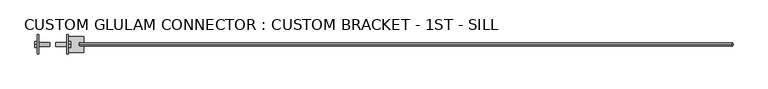
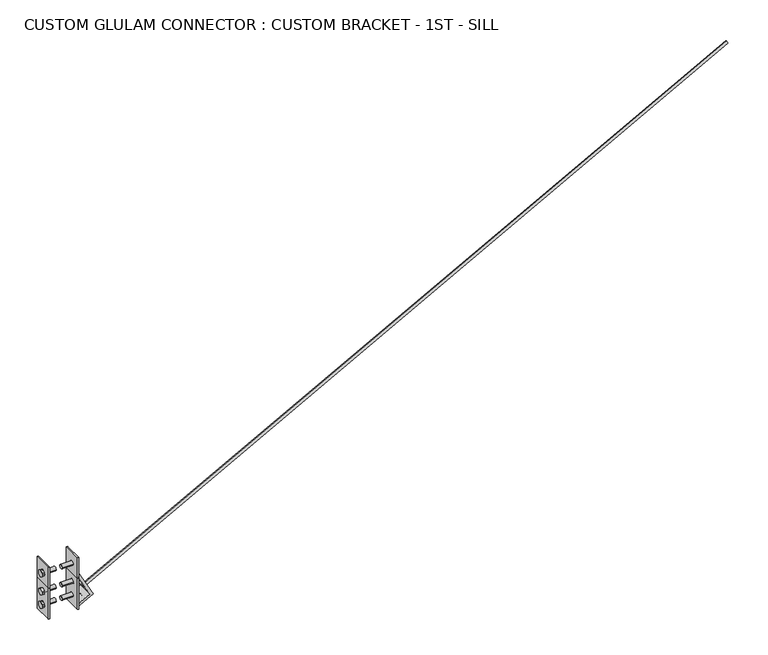
"""IFC4 building model written with IfcOpenShell, lengths in millimetres: fastener geometry, CUSTOM GLULAM CONNECTOR : CUSTOM BRACKET - 1ST - SILL."""

import ifcopenshell
import ifcopenshell.guid

model = None  # the IFC model being written
_history = None  # IfcOwnerHistory: only IFC2X3 demands one
_inside = {}  # id of a spatial element -> (the spatial element, [elements in it])
_under = {}  # id of a project, library or spatial element -> (it, [spatial elements below it])
_declared = {}  # id of a project -> (the project, [libraries it declares])
_typed = {}  # id of a type object -> (the type object, [elements of that type])
_made_of = {}  # id of a material, layer set ... -> (it, [elements and type objects made of it])


def new_model(schema):
    """Start an empty IFC model of exactly this schema.

    Asked for "IFC4X3", IfcOpenShell would pick the latest addendum, in which some entities
    have other attributes; the version numbers below select the first issue.
    IFC2X3 requires an IfcOwnerHistory on every rooted entity: one is made here for all.
    """
    global model, _history
    if schema == "IFC4X3":
        model = ifcopenshell.file(schema_version=(4, 3, 0, 0))
    else:
        model = ifcopenshell.file(schema=schema)
    _inside.clear()
    _under.clear()
    _declared.clear()
    _typed.clear()
    _made_of.clear()
    _history = None
    if model.schema == "IFC2X3":
        org = make("IfcOrganization", Name="unknown")
        user = make(
            "IfcPersonAndOrganization",
            ThePerson=make("IfcPerson", FamilyName="unknown"),
            TheOrganization=org,
        )
        app = make(
            "IfcApplication",
            ApplicationDeveloper=org,
            Version="unknown",
            ApplicationFullName="unknown",
            ApplicationIdentifier="unknown",
        )
        _history = make(
            "IfcOwnerHistory",
            OwningUser=user,
            OwningApplication=app,
            ChangeAction="ADDED",
            CreationDate=0,
        )
    return model


def make(cls, **values):
    """One entity of the class cls with the attributes given. An attribute that is None is left unset."""
    return model.create_entity(
        cls, **{name: value for name, value in values.items() if value is not None}
    )


def rooted(cls, **values):
    """An entity with a GlobalId (a new one), such as an element, a storey or a relation."""
    return make(cls, GlobalId=ifcopenshell.guid.new(), OwnerHistory=_history, **values)


def si_unit(unit_type, name, prefix=None):
    """IfcSIUnit, for example si_unit("LENGTHUNIT", "METRE", prefix="MILLI")."""
    return make("IfcSIUnit", UnitType=unit_type, Prefix=prefix, Name=name)


def assignment(units):
    """IfcUnitAssignment: the units of a project."""
    return None if units is None else make("IfcUnitAssignment", Units=units)


def point(xyz):
    """IfcCartesianPoint."""
    return None if xyz is None else make("IfcCartesianPoint", Coordinates=xyz)


def direction(xyz):
    """IfcDirection."""
    return None if xyz is None else make("IfcDirection", DirectionRatios=xyz)


def frame(location, z_axis=None, x_axis=None):
    """IfcAxis2Placement3D, a coordinate frame: its origin and axes. An axis left out is left unset."""
    return make(
        "IfcAxis2Placement3D",
        Location=point(location),
        Axis=direction(z_axis),
        RefDirection=direction(x_axis),
    )


def frame_2d(location, x_axis=None):
    """IfcAxis2Placement2D, a coordinate frame in the plane: its origin and x axis."""
    return make(
        "IfcAxis2Placement2D", Location=point(location), RefDirection=direction(x_axis)
    )


def origin():
    """The frame at (0, 0, 0) with its axes left unset."""
    return frame((0.0, 0.0, 0.0))


def place(relative_to, where):
    """IfcLocalPlacement: puts the frame where relative to a parent placement (None: the world)."""
    return make(
        "IfcLocalPlacement", PlacementRelTo=relative_to, RelativePlacement=where
    )


def context(
    kind, dimensions, precision=None, world=None, true_north=None, identifier=None
):
    """IfcGeometricRepresentationContext, for example the 3D "Model" context."""
    return make(
        "IfcGeometricRepresentationContext",
        ContextIdentifier=identifier,
        ContextType=kind,
        CoordinateSpaceDimension=dimensions,
        Precision=precision,
        WorldCoordinateSystem=world,
        TrueNorth=true_north,
    )


def project(units=None, contexts=None):
    """IfcProject with its units and contexts."""
    return rooted(
        "IfcProject",
        Name="project",
        RepresentationContexts=contexts,
        UnitsInContext=assignment(units),
    )


def spatial(cls, under=None, at=None, **own):
    """A site, building, storey or space (cls), placed at a placement, below another one or the project."""
    s = rooted(cls, ObjectPlacement=at, **own)
    if under is not None:
        _under.setdefault(under.id(), (under, []))[1].append(s)
    return s


def polyline(points):
    """IfcPolyline through the points."""
    return make("IfcPolyline", Points=[point(p) for p in points])


def circle_curve(where, radius):
    """IfcCircle in the frame where."""
    return make("IfcCircle", Position=where, Radius=radius)


def trimmed(basis, trim1, trim2, sense, master):
    """IfcTrimmedCurve: the piece of a basis curve between two trims."""
    return make(
        "IfcTrimmedCurve",
        BasisCurve=basis,
        Trim1=trim1,
        Trim2=trim2,
        SenseAgreement=sense,
        MasterRepresentation=master,
    )


def segment(curve, same_sense, transition):
    """IfcCompositeCurveSegment."""
    return make(
        "IfcCompositeCurveSegment",
        Transition=transition,
        SameSense=same_sense,
        ParentCurve=curve,
    )


def composite_curve(segments, self_intersect=None):
    """IfcCompositeCurve: segments joined end to end."""
    return make("IfcCompositeCurve", Segments=segments, SelfIntersect=self_intersect)


def outline(outer, holes=None, kind="AREA"):
    """IfcArbitraryClosedProfileDef: a profile drawn as a closed curve; with holes, ...WithVoids."""
    if holes is None:
        return make("IfcArbitraryClosedProfileDef", ProfileType=kind, OuterCurve=outer)
    return make(
        "IfcArbitraryProfileDefWithVoids",
        ProfileType=kind,
        OuterCurve=outer,
        InnerCurves=holes,
    )


def extrude(swept, where, along, depth):
    """IfcExtrudedAreaSolid: the profile swept, set in the frame where, extruded along a direction by depth."""
    return make(
        "IfcExtrudedAreaSolid",
        SweptArea=swept,
        Position=where,
        ExtrudedDirection=direction(along),
        Depth=depth,
    )


def shape(context_of_items, identifier, shape_type, items):
    """IfcShapeRepresentation: the items that make up one representation, for example the "Body"."""
    return make(
        "IfcShapeRepresentation",
        ContextOfItems=context_of_items,
        RepresentationIdentifier=identifier,
        RepresentationType=shape_type,
        Items=items,
    )


def source(mapping_origin, context_of_items, identifier, shape_type, items):
    """IfcRepresentationMap: a shape defined once, which mapped items show again and again."""
    return make(
        "IfcRepresentationMap",
        MappingOrigin=mapping_origin,
        MappedRepresentation=shape(context_of_items, identifier, shape_type, items),
    )


def transform(
    local_origin,
    x_axis=None,
    y_axis=None,
    z_axis=None,
    scale=None,
    scale2=None,
    scale3=None,
    uniform=True,
):
    """IfcCartesianTransformationOperator3D, or its non-uniform kind. x_axis, y_axis, z_axis: its Axis1, 2, 3."""
    if uniform:
        return make(
            "IfcCartesianTransformationOperator3D",
            Axis1=direction(x_axis),
            Axis2=direction(y_axis),
            LocalOrigin=point(local_origin),
            Scale=scale,
            Axis3=direction(z_axis),
        )
    return make(
        "IfcCartesianTransformationOperator3DnonUniform",
        Axis1=direction(x_axis),
        Axis2=direction(y_axis),
        LocalOrigin=point(local_origin),
        Scale=scale,
        Axis3=direction(z_axis),
        Scale2=scale2,
        Scale3=scale3,
    )


def mapped(mapping_source, mapping_target):
    """IfcMappedItem: shows the shape of a source again, moved by a transform."""
    return make(
        "IfcMappedItem", MappingSource=mapping_source, MappingTarget=mapping_target
    )


def made_of(thing, what):
    """Note that an element or type object is made of a material, layer set ...; save() writes the relation."""
    if what is not None:
        _made_of.setdefault(what.id(), (what, []))[1].append(thing)
    return thing


def element(
    cls,
    number,
    at=None,
    inside=None,
    cuts=None,
    type_object=None,
    material=None,
    context=None,
    identifier="Body",
    shape_type=None,
    held_by="IfcProductDefinitionShape",
    body=None,
    shapes=None,
    **own,
):
    """One element of the class cls, such as IfcWall. Its Tag is "e" and its number.

    at: its placement. inside: the storey or other place that contains it. cuts: it is an
    opening in that element (IfcRelVoidsElement). A single representation is given by context,
    identifier, shape_type and body (its items); several are given by shapes. held_by: the class
    of the entity that holds the representations. save() writes the other relations.
    """
    e = rooted(cls, Tag="e%d" % number, ObjectPlacement=at, **own)
    if body is not None:
        shapes = [shape(context, identifier, shape_type, body)]
    if shapes is not None:
        e.Representation = make(held_by, Representations=shapes)
    if inside is not None:
        _inside.setdefault(inside.id(), (inside, []))[1].append(e)
    if cuts is not None:
        rooted(
            "IfcRelVoidsElement", RelatingBuildingElement=cuts, RelatedOpeningElement=e
        )
    if type_object is not None:
        _typed.setdefault(type_object.id(), (type_object, []))[1].append(e)
    return made_of(e, material)


def aggregate(whole, parts):
    """IfcRelAggregates: a whole, such as a stair, and the parts it consists of."""
    return rooted("IfcRelAggregates", RelatingObject=whole, RelatedObjects=parts)


def save(model, path):
    """Write the relations noted so far, then the file.

    IfcRelAggregates (storeys below a building ...), IfcRelContainedInSpatialStructure (elements
    in a storey), IfcRelDefinesByType, IfcRelAssociatesMaterial and IfcRelDeclares: one each for
    every whole, place, type object, material and project.
    """
    for whole, parts in _under.values():
        aggregate(whole, parts)
    for where, things in _inside.values():
        rooted(
            "IfcRelContainedInSpatialStructure",
            RelatedElements=things,
            RelatingStructure=where,
        )
    for kind, things in _typed.values():
        rooted("IfcRelDefinesByType", RelatedObjects=things, RelatingType=kind)
    for what, things in _made_of.values():
        rooted("IfcRelAssociatesMaterial", RelatedObjects=things, RelatingMaterial=what)
    for by, libraries in _declared.values():
        rooted("IfcRelDeclares", RelatingContext=by, RelatedDefinitions=libraries)
    model.write(path)


def plane_surface(at):
    """IfcPlane: the flat surface through the origin of the frame at, square to its z axis."""
    return make("IfcPlane", Position=at)


def revolved_surface(curve, axis_point, axis_direction):
    """IfcSurfaceOfRevolution: the curve turned about the line through axis_point along axis_direction."""
    return make(
        "IfcSurfaceOfRevolution",
        SweptCurve=make("IfcArbitraryOpenProfileDef", ProfileType="CURVE", Curve=curve),
        AxisPosition=make("IfcAxis1Placement", Location=point(axis_point), Axis=direction(axis_direction)),
    )


def advanced_brep(points, edges, surfaces, faces):
    """IfcAdvancedBrep: a solid bounded by faces that lie on surfaces and meet in shared edges.

    An edge is (start, end): straight between two places in points (the first is 0);
    or (start, end, curve); or (start, end, curve, False) where it runs against its curve.
    A face is (place in surfaces, loops), or (place, loops, False) where it looks against
    its surface's normal. A loop lists edges by number (the first is 1), with a minus sign
    where the edge is run from its end to its start. The first loop is the outer one.
    """
    corners = [point(p) for p in points]
    vertices = [make("IfcVertexPoint", VertexGeometry=c) for c in corners]
    made = []
    for start, end, *more in edges:
        made.append(
            make(
                "IfcEdgeCurve",
                EdgeStart=vertices[start],
                EdgeEnd=vertices[end],
                EdgeGeometry=more[0] if more else make("IfcPolyline", Points=[corners[start], corners[end]]),
                SameSense=more[1] if len(more) > 1 else True,
            )
        )
    hull = []
    for where, loops, *sense in faces:
        bounds = []
        for j, loop in enumerate(loops):
            ring = [make("IfcOrientedEdge", EdgeElement=made[abs(k) - 1], Orientation=k > 0) for k in loop]
            bounds.append(
                make(
                    "IfcFaceOuterBound" if j == 0 else "IfcFaceBound",
                    Bound=make("IfcEdgeLoop", EdgeList=ring),
                    Orientation=True,
                )
            )
        hull.append(make("IfcAdvancedFace", Bounds=bounds, FaceSurface=surfaces[where], SameSense=sense[0] if sense else True))
    return make("IfcAdvancedBrep", Outer=make("IfcClosedShell", CfsFaces=hull))


def custom_glulam_connector_custom_bracket_1st_sill_41cb3a86(model_context):
    return source(origin(), model_context, "Body", "SolidModel", [
        advanced_brep(
        [(-87.3125, 13.890625, 160.3375), (-95.25, 13.890625, 160.3375), (-95.25, -13.890625, 160.3375), (-87.3125, -13.890625, 160.3375), (-95.25, -60.325, 211.1375), (-95.25, -52.3875, 211.1375), (-95.25, 60.325, 211.1375), (-95.25, 60.325, 7.9375), (-95.25, -52.3875, 7.9375), (-95.25, -60.325, 7.9375), (-95.25, -13.890625, 71.4375), (-95.25, 13.890625, 71.4375), (-87.3125, 13.890625, 71.4375), (-87.3125, -13.890625, 71.4375), (-87.3125, -60.325, 211.1375), (-87.3125, -60.325, 7.9375), (-87.3125, 60.325, 7.9375), (-87.3125, 60.325, 211.1375)],
        [
            (0, 1),
            (1, 2, circle_curve(frame((-95.25, 0.0, 160.3375), z_axis=(-1.0, 0.0, 0.0), x_axis=(0.0, -1.0, 0.0)), 13.890625)),
            (2, 3),
            (3, 0, circle_curve(frame((-87.3125, 0.0, 160.3375), z_axis=(1.0, 0.0, 0.0), x_axis=(0.0, -1.0, 0.0)), 13.890625)),
            (4, 5),
            (5, 6),
            (6, 7),
            (7, 8),
            (8, 9),
            (9, 4),
            (1, 2, circle_curve(frame((-95.25, 0.0, 160.3375), z_axis=(1.0, 0.0, 0.0), x_axis=(0.0, -1.0, 0.0)), 13.890625)),
            (10, 11, circle_curve(frame((-95.25, 0.0, 71.4375), z_axis=(1.0, 0.0, 0.0), x_axis=(0.0, -1.0, 0.0)), 13.890625)),
            (11, 10, circle_curve(frame((-95.25, 0.0, 71.4375), z_axis=(1.0, 0.0, 0.0), x_axis=(0.0, -1.0, 0.0)), 13.890625)),
            (11, 12),
            (12, 13, circle_curve(frame((-87.3125, 0.0, 71.4375), z_axis=(1.0, 0.0, 0.0), x_axis=(0.0, -1.0, 0.0)), 13.890625)),
            (13, 10),
            (0, 3, circle_curve(frame((-87.3125, 0.0, 160.3375), z_axis=(1.0, 0.0, 0.0), x_axis=(0.0, -1.0, 0.0)), 13.890625)),
            (13, 12, circle_curve(frame((-87.3125, 0.0, 71.4375), z_axis=(1.0, 0.0, 0.0), x_axis=(0.0, -1.0, 0.0)), 13.890625)),
            (14, 15),
            (15, 16),
            (16, 17),
            (17, 14),
            (4, 14),
            (17, 6),
            (16, 7),
            (15, 9),
        ],
        [
            revolved_surface(polyline([(-95.25, -13.890625, 160.3375), (-87.3125, -13.890625, 160.3375)]), (-87.3125, 0.0, 160.3375), (-1.0, 0.0, 0.0)),
            plane_surface(frame((-95.25, 60.325, 211.1375), z_axis=(-1.0, 0.0, 0.0), x_axis=(0.0, 1.0, 0.0))),
            revolved_surface(polyline([(-95.25, -13.890625, 71.4375), (-87.3125, -13.890625, 71.4375)]), (-87.3125, 0.0, 71.4375), (-1.0, 0.0, 0.0)),
            plane_surface(frame((-87.3125, 60.325, 211.1375), z_axis=(1.0, 0.0, 0.0), x_axis=(0.0, -1.0, 0.0))),
            plane_surface(frame((-95.25, -60.325, 211.1375), z_axis=(0.0, 0.0, 1.0), x_axis=(1.0, 0.0, 0.0))),
            plane_surface(frame((-95.25, 60.325, 211.1375), z_axis=(0.0, 1.0, 0.0), x_axis=(1.0, 0.0, 0.0))),
            plane_surface(frame((-95.25, 60.325, 7.9375), z_axis=(0.0, 0.0, -1.0), x_axis=(1.0, 0.0, 0.0))),
            plane_surface(frame((-95.25, -60.325, 7.9375), z_axis=(0.0, -1.0, 0.0), x_axis=(1.0, 0.0, 0.0))),
        ],
        [
            (0, [[1, 2, 3, 4]]),
            (1, [[5, 6, 7, 8, 9, 10], [-2, 11], [12, 13]]),
            (2, [[14, 15, 16, -13]]),
            (0, [[-1, 17, -3, -11]]),
            (2, [[-14, -12, -16, 18]]),
            (3, [[19, 20, 21, 22], [-4, -17], [-18, -15]]),
            (4, [[-6, -5, 23, -22, 24]]),
            (5, [[-7, -24, -21, 25]]),
            (6, [[-9, -8, -25, -20, 26]]),
            (7, [[-10, -26, -19, -23]]),
        ],
    ),
        extrude(outline(polyline([(19.05, 171.3360226), (19.05, 149.3389774), (0.0, 138.3404547), (-19.05, 149.3389774), (-19.05, 171.3360226), (0.0, 182.3345453), (19.05, 171.3360226)])), frame((-110.2320312, 0.0, 0.0), z_axis=(1.0, 0.0, 0.0), x_axis=(0.0, 1.0, 0.0)), (0.0, 0.0, 1.0), 14.9820312),
        extrude(outline(composite_curve([segment(trimmed(circle_curve(frame_2d((0.0, 160.3375)), 12.7), [point((12.7, 160.3375))], [point((-12.7, 160.3375))], False, "CARTESIAN"), True, "CONTINUOUS"), segment(trimmed(circle_curve(frame_2d((0.0, 160.3375)), 12.7), [point((-12.7, 160.3375))], [point((12.7, 160.3375))], False, "CARTESIAN"), True, "CONTINUOUS")], self_intersect=False)), frame((-95.25, 0.0, 0.0), z_axis=(1.0, 0.0, 0.0), x_axis=(0.0, 1.0, 0.0)), (0.0, 0.0, 1.0), 76.2),
        extrude(outline(polyline([(19.05, 82.4360226), (19.05, 60.4389774), (0.0, 49.4404547), (-19.05, 60.4389774), (-19.05, 82.4360226), (0.0, 93.4345453), (19.05, 82.4360226)])), frame((-110.2320312, 0.0, 0.0), z_axis=(1.0, 0.0, 0.0), x_axis=(0.0, 1.0, 0.0)), (0.0, 0.0, 1.0), 14.9820312),
        extrude(outline(composite_curve([segment(trimmed(circle_curve(frame_2d((0.0, 71.4375)), 12.7), [point((12.7, 71.4375))], [point((-12.7, 71.4375))], False, "CARTESIAN"), True, "CONTINUOUS"), segment(trimmed(circle_curve(frame_2d((0.0, 71.4375)), 12.7), [point((-12.7, 71.4375))], [point((12.7, 71.4375))], False, "CARTESIAN"), True, "CONTINUOUS")], self_intersect=False)), frame((-95.25, 0.0, 0.0), z_axis=(1.0, 0.0, 0.0), x_axis=(0.0, 1.0, 0.0)), (0.0, 0.0, 1.0), 76.2),
        extrude(outline(polyline([(19.05, 171.3360226), (19.05, 149.3389774), (0.0, 138.3404547), (-19.05, 149.3389774), (-19.05, 171.3360226), (0.0, 182.3345453), (19.05, 171.3360226)])), frame((-110.2320312, 0.0, 0.0), z_axis=(1.0, 0.0, 0.0), x_axis=(0.0, 1.0, 0.0)), (0.0, 0.0, 1.0), 14.9820312),
        extrude(outline(composite_curve([segment(trimmed(circle_curve(frame_2d((0.0, 160.3375)), 12.7), [point((12.7, 160.3375))], [point((-12.7, 160.3375))], False, "CARTESIAN"), True, "CONTINUOUS"), segment(trimmed(circle_curve(frame_2d((0.0, 160.3375)), 12.7), [point((-12.7, 160.3375))], [point((12.7, 160.3375))], False, "CARTESIAN"), True, "CONTINUOUS")], self_intersect=False)), frame((-95.25, 0.0, 0.0), z_axis=(1.0, 0.0, 0.0), x_axis=(0.0, 1.0, 0.0)), (0.0, 0.0, 1.0), 76.2),
        extrude(outline(polyline([(19.05, 171.3360226), (19.05, 149.3389774), (0.0, 138.3404547), (-19.05, 149.3389774), (-19.05, 171.3360226), (0.0, 182.3345453), (19.05, 171.3360226)])), frame((95.25, 0.0, 0.0), z_axis=(1.0, 0.0, 0.0), x_axis=(0.0, 1.0, 0.0)), (0.0, 0.0, 1.0), 14.9820312),
        extrude(outline(composite_curve([segment(trimmed(circle_curve(frame_2d((0.0, 160.3375)), 12.7), [point((12.7, 160.3375))], [point((-12.7, 160.3375))], False, "CARTESIAN"), True, "CONTINUOUS"), segment(trimmed(circle_curve(frame_2d((0.0, 160.3375)), 12.7), [point((-12.7, 160.3375))], [point((12.7, 160.3375))], False, "CARTESIAN"), True, "CONTINUOUS")], self_intersect=False)), frame((19.05, 0.0, 0.0), z_axis=(1.0, 0.0, 0.0), x_axis=(0.0, 1.0, 0.0)), (0.0, 0.0, 1.0), 76.2),
        extrude(outline(polyline([(19.05, 82.4360226), (19.05, 60.4389774), (0.0, 49.4404547), (-19.05, 60.4389774), (-19.05, 82.4360226), (0.0, 93.4345453), (19.05, 82.4360226)])), frame((95.25, 0.0, 0.0), z_axis=(1.0, 0.0, 0.0), x_axis=(0.0, 1.0, 0.0)), (0.0, 0.0, 1.0), 14.9820312),
        extrude(outline(composite_curve([segment(trimmed(circle_curve(frame_2d((0.0, 71.4375)), 12.7), [point((12.7, 71.4375))], [point((-12.7, 71.4375))], False, "CARTESIAN"), True, "CONTINUOUS"), segment(trimmed(circle_curve(frame_2d((0.0, 71.4375)), 12.7), [point((-12.7, 71.4375))], [point((12.7, 71.4375))], False, "CARTESIAN"), True, "CONTINUOUS")], self_intersect=False)), frame((19.05, 0.0, 0.0), z_axis=(1.0, 0.0, 0.0), x_axis=(0.0, 1.0, 0.0)), (0.0, 0.0, 1.0), 76.2),
        extrude(outline(polyline([(19.05, 171.3360226), (19.05, 149.3389774), (0.0, 138.3404547), (-19.05, 149.3389774), (-19.05, 171.3360226), (0.0, 182.3345453), (19.05, 171.3360226)])), frame((95.25, 0.0, 0.0), z_axis=(1.0, 0.0, 0.0), x_axis=(0.0, 1.0, 0.0)), (0.0, 0.0, 1.0), 14.9820312),
        extrude(outline(composite_curve([segment(trimmed(circle_curve(frame_2d((0.0, 160.3375)), 12.7), [point((12.7, 160.3375))], [point((-12.7, 160.3375))], False, "CARTESIAN"), True, "CONTINUOUS"), segment(trimmed(circle_curve(frame_2d((0.0, 160.3375)), 12.7), [point((-12.7, 160.3375))], [point((12.7, 160.3375))], False, "CARTESIAN"), True, "CONTINUOUS")], self_intersect=False)), frame((19.05, 0.0, 0.0), z_axis=(1.0, 0.0, 0.0), x_axis=(0.0, 1.0, 0.0)), (0.0, 0.0, 1.0), 76.2),
        advanced_brep(
        [(87.3125, 13.890625, 160.3375), (87.3125, -13.890625, 160.3375), (95.25, -13.890625, 160.3375), (95.25, 13.890625, 160.3375), (95.25, -60.325, 211.1375), (95.25, -60.325, 7.9375), (95.25, -52.3875, 7.9375), (95.25, 60.325, 7.9375), (95.25, 60.325, 211.1375), (95.25, -52.3875, 211.1375), (95.25, -13.890625, 71.4375), (95.25, 13.890625, 71.4375), (87.3125, -13.890625, 71.4375), (87.3125, 13.890625, 71.4375), (87.3125, -60.325, 211.1375), (87.3125, 60.325, 211.1375), (87.3125, 60.325, 7.9375), (87.3125, -60.325, 7.9375)],
        [
            (0, 1, circle_curve(frame((87.3125, 0.0, 160.3375), z_axis=(-1.0, 0.0, 0.0), x_axis=(0.0, -1.0, 0.0)), 13.890625)),
            (1, 2),
            (2, 3, circle_curve(frame((95.25, 0.0, 160.3375), z_axis=(1.0, 0.0, 0.0), x_axis=(0.0, -1.0, 0.0)), 13.890625)),
            (3, 0),
            (4, 5),
            (5, 6),
            (6, 7),
            (7, 8),
            (8, 9),
            (9, 4),
            (10, 11, circle_curve(frame((95.25, 0.0, 71.4375), z_axis=(-1.0, 0.0, 0.0), x_axis=(0.0, -1.0, 0.0)), 13.890625)),
            (11, 10, circle_curve(frame((95.25, 0.0, 71.4375), z_axis=(-1.0, 0.0, 0.0), x_axis=(0.0, -1.0, 0.0)), 13.890625)),
            (2, 3, circle_curve(frame((95.25, 0.0, 160.3375), z_axis=(-1.0, 0.0, 0.0), x_axis=(0.0, -1.0, 0.0)), 13.890625)),
            (10, 12),
            (12, 13, circle_curve(frame((87.3125, 0.0, 71.4375), z_axis=(-1.0, 0.0, 0.0), x_axis=(0.0, -1.0, 0.0)), 13.890625)),
            (13, 11),
            (1, 0, circle_curve(frame((87.3125, 0.0, 160.3375), z_axis=(-1.0, 0.0, 0.0), x_axis=(0.0, -1.0, 0.0)), 13.890625)),
            (13, 12, circle_curve(frame((87.3125, 0.0, 71.4375), z_axis=(-1.0, 0.0, 0.0), x_axis=(0.0, -1.0, 0.0)), 13.890625)),
            (14, 15),
            (15, 16),
            (16, 17),
            (17, 14),
            (8, 15),
            (14, 4),
            (7, 16),
            (5, 17),
        ],
        [
            revolved_surface(polyline([(95.25, -13.890625, 160.3375), (87.3125, -13.890625, 160.3375)]), (87.3125, 0.0, 160.3375), (1.0, 0.0, 0.0)),
            plane_surface(frame((95.25, 60.325, 211.1375), z_axis=(1.0, 0.0, 0.0), x_axis=(0.0, 1.0, 0.0))),
            revolved_surface(polyline([(95.25, -13.890625, 71.4375), (87.3125, -13.890625, 71.4375)]), (87.3125, 0.0, 71.4375), (1.0, 0.0, 0.0)),
            plane_surface(frame((87.3125, 60.325, 211.1375), z_axis=(-1.0, 0.0, 0.0), x_axis=(0.0, -1.0, 0.0))),
            plane_surface(frame((95.25, -60.325, 211.1375), z_axis=(0.0, 0.0, 1.0), x_axis=(-1.0, 0.0, 0.0))),
            plane_surface(frame((95.25, 60.325, 211.1375), z_axis=(0.0, 1.0, 0.0), x_axis=(-1.0, 0.0, 0.0))),
            plane_surface(frame((95.25, 60.325, 7.9375), z_axis=(0.0, 0.0, -1.0), x_axis=(-1.0, 0.0, 0.0))),
            plane_surface(frame((95.25, -60.325, 7.9375), z_axis=(0.0, -1.0, 0.0), x_axis=(-1.0, 0.0, 0.0))),
        ],
        [
            (0, [[1, 2, 3, 4]]),
            (1, [[5, 6, 7, 8, 9, 10], [11, 12], [13, -3]]),
            (2, [[-11, 14, 15, 16]]),
            (0, [[-13, -2, 17, -4]]),
            (2, [[18, -14, -12, -16]]),
            (3, [[19, 20, 21, 22], [-17, -1], [-15, -18]]),
            (4, [[23, -19, 24, -10, -9]]),
            (5, [[25, -20, -23, -8]]),
            (6, [[26, -21, -25, -7, -6]]),
            (7, [[-24, -22, -26, -5]]),
        ],
    ),
        extrude(outline(polyline([(19.05, 291.9860226), (19.05, 269.9889774), (0.0, 258.9904547), (-19.05, 269.9889774), (-19.05, 291.9860226), (0.0, 302.9845453), (19.05, 291.9860226)])), frame((-110.2320312, 0.0, 0.0), z_axis=(1.0, 0.0, 0.0), x_axis=(0.0, 1.0, 0.0)), (0.0, 0.0, 1.0), 14.9820312),
        extrude(outline(composite_curve([segment(trimmed(circle_curve(frame_2d((0.0, 280.9875)), 12.7), [point((12.7, 280.9875))], [point((-12.7, 280.9875))], False, "CARTESIAN"), True, "CONTINUOUS"), segment(trimmed(circle_curve(frame_2d((0.0, 280.9875)), 12.7), [point((-12.7, 280.9875))], [point((12.7, 280.9875))], False, "CARTESIAN"), True, "CONTINUOUS")], self_intersect=False)), frame((-95.25, 0.0, 0.0), z_axis=(1.0, 0.0, 0.0), x_axis=(0.0, 1.0, 0.0)), (0.0, 0.0, 1.0), 76.2),
        advanced_brep(
        [(-95.25, -60.325, 350.8375), (-95.25, -60.325, 211.1375), (-87.3125, -60.325, 211.1375), (-87.3125, -60.325, 350.8375), (-87.3125, 13.890625, 280.9875), (-95.25, 13.890625, 280.9875), (-95.25, -13.890625, 280.9875), (-87.3125, -13.890625, 280.9875), (-95.25, 60.325, 350.8375), (-95.25, 52.3875, 350.8375), (-87.3125, 60.325, 350.8375), (-95.25, 60.325, 211.1375), (-95.25, 52.3875, 211.1375), (-87.3125, 60.325, 211.1375)],
        [
            (0, 1),
            (1, 2),
            (2, 3),
            (3, 0),
            (4, 5),
            (5, 6, circle_curve(frame((-95.25, 0.0, 280.9875), z_axis=(-1.0, 0.0, 0.0), x_axis=(0.0, -1.0, 0.0)), 13.890625)),
            (6, 7),
            (7, 4, circle_curve(frame((-87.3125, 0.0, 280.9875), z_axis=(1.0, 0.0, 0.0), x_axis=(0.0, -1.0, 0.0)), 13.890625)),
            (4, 7, circle_curve(frame((-87.3125, 0.0, 280.9875), z_axis=(1.0, 0.0, 0.0), x_axis=(0.0, -1.0, 0.0)), 13.890625)),
            (6, 5, circle_curve(frame((-95.25, 0.0, 280.9875), z_axis=(-1.0, 0.0, 0.0), x_axis=(0.0, -1.0, 0.0)), 13.890625)),
            (8, 9),
            (9, 0),
            (3, 10),
            (10, 8),
            (8, 11),
            (11, 12),
            (12, 1),
            (2, 13),
            (13, 10),
            (13, 11),
        ],
        [
            plane_surface(frame((-95.25, -60.325, 211.1375), z_axis=(0.0, -1.0, 0.0), x_axis=(1.0, 0.0, 0.0))),
            revolved_surface(polyline([(-95.25, -13.890625, 280.9875), (-87.3125, -13.890625, 280.9875)]), (-87.3125, 0.0, 280.9875), (-1.0, 0.0, 0.0)),
            plane_surface(frame((-95.25, -60.325, 350.8375), z_axis=(0.0, 0.0, 1.0), x_axis=(1.0, 0.0, 0.0))),
            plane_surface(frame((-95.25, 60.325, 350.8375), z_axis=(-1.0, 0.0, 0.0), x_axis=(0.0, 1.0, 0.0))),
            plane_surface(frame((-87.3125, 60.325, 350.8375), z_axis=(1.0, 0.0, 0.0), x_axis=(0.0, -1.0, 0.0))),
            plane_surface(frame((-95.25, 60.325, 350.8375), z_axis=(0.0, 1.0, 0.0), x_axis=(1.0, 0.0, 0.0))),
            plane_surface(frame((-95.25, 60.325, 211.1375), z_axis=(0.0, 0.0, -1.0), x_axis=(1.0, 0.0, 0.0))),
        ],
        [
            (0, [[1, 2, 3, 4]]),
            (1, [[5, 6, 7, 8]]),
            (1, [[-5, 9, -7, 10]]),
            (2, [[11, 12, -4, 13, 14]]),
            (3, [[-12, -11, 15, 16, 17, -1], [-6, -10]]),
            (4, [[-3, 18, 19, -13], [-8, -9]]),
            (5, [[-15, -14, -19, 20]]),
            (6, [[-17, -16, -20, -18, -2]]),
        ],
    ),
        advanced_brep(
        [(95.25, -60.325, 350.8375), (87.3125, -60.325, 350.8375), (87.3125, -60.325, 211.1375), (95.25, -60.325, 211.1375), (87.3125, 13.890625, 280.9875), (87.3125, -13.890625, 280.9875), (95.25, -13.890625, 280.9875), (95.25, 13.890625, 280.9875), (95.25, 60.325, 350.8375), (87.3125, 60.325, 350.8375), (95.25, 52.3875, 350.8375), (95.25, 52.3875, 211.1375), (95.25, 60.325, 211.1375), (87.3125, 60.325, 211.1375)],
        [
            (0, 1),
            (1, 2),
            (2, 3),
            (3, 0),
            (4, 5, circle_curve(frame((87.3125, 0.0, 280.9875), z_axis=(-1.0, 0.0, 0.0), x_axis=(0.0, -1.0, 0.0)), 13.890625)),
            (5, 6),
            (6, 7, circle_curve(frame((95.25, 0.0, 280.9875), z_axis=(1.0, 0.0, 0.0), x_axis=(0.0, -1.0, 0.0)), 13.890625)),
            (7, 4),
            (7, 6, circle_curve(frame((95.25, 0.0, 280.9875), z_axis=(1.0, 0.0, 0.0), x_axis=(0.0, -1.0, 0.0)), 13.890625)),
            (5, 4, circle_curve(frame((87.3125, 0.0, 280.9875), z_axis=(-1.0, 0.0, 0.0), x_axis=(0.0, -1.0, 0.0)), 13.890625)),
            (8, 9),
            (9, 1),
            (0, 10),
            (10, 8),
            (3, 11),
            (11, 12),
            (12, 8),
            (9, 13),
            (13, 2),
            (12, 13),
        ],
        [
            plane_surface(frame((95.25, -60.325, 211.1375), z_axis=(0.0, -1.0, 0.0), x_axis=(-1.0, 0.0, 0.0))),
            revolved_surface(polyline([(95.25, -13.890625, 280.9875), (87.3125, -13.890625, 280.9875)]), (87.3125, 0.0, 280.9875), (1.0, 0.0, 0.0)),
            plane_surface(frame((95.25, -60.325, 350.8375), z_axis=(0.0, 0.0, 1.0), x_axis=(-1.0, 0.0, 0.0))),
            plane_surface(frame((95.25, 60.325, 350.8375), z_axis=(1.0, 0.0, 0.0), x_axis=(0.0, 1.0, 0.0))),
            plane_surface(frame((87.3125, 60.325, 350.8375), z_axis=(-1.0, 0.0, 0.0), x_axis=(0.0, -1.0, 0.0))),
            plane_surface(frame((95.25, 60.325, 350.8375), z_axis=(0.0, 1.0, 0.0), x_axis=(-1.0, 0.0, 0.0))),
            plane_surface(frame((95.25, 60.325, 211.1375), z_axis=(0.0, 0.0, -1.0), x_axis=(-1.0, 0.0, 0.0))),
        ],
        [
            (0, [[1, 2, 3, 4]]),
            (1, [[5, 6, 7, 8]]),
            (1, [[9, -6, 10, -8]]),
            (2, [[11, 12, -1, 13, 14]]),
            (3, [[-4, 15, 16, 17, -14, -13], [-9, -7]]),
            (4, [[-12, 18, 19, -2], [-10, -5]]),
            (5, [[20, -18, -11, -17]]),
            (6, [[-3, -19, -20, -16, -15]]),
        ],
    ),
        extrude(outline(polyline([(19.05, 291.9860226), (19.05, 269.9889774), (0.0, 258.9904547), (-19.05, 269.9889774), (-19.05, 291.9860226), (0.0, 302.9845453), (19.05, 291.9860226)])), frame((95.25, 0.0, 0.0), z_axis=(1.0, 0.0, 0.0), x_axis=(0.0, 1.0, 0.0)), (0.0, 0.0, 1.0), 14.9820312),
        extrude(outline(composite_curve([segment(trimmed(circle_curve(frame_2d((0.0, 280.9875)), 12.7), [point((12.7, 280.9875))], [point((-12.7, 280.9875))], False, "CARTESIAN"), True, "CONTINUOUS"), segment(trimmed(circle_curve(frame_2d((0.0, 280.9875)), 12.7), [point((-12.7, 280.9875))], [point((12.7, 280.9875))], False, "CARTESIAN"), True, "CONTINUOUS")], self_intersect=False)), frame((19.05, 0.0, 0.0), z_axis=(1.0, 0.0, 0.0), x_axis=(0.0, 1.0, 0.0)), (0.0, 0.0, 1.0), 76.2),
        extrude(outline(composite_curve([segment(trimmed(circle_curve(frame_2d((0.0, 9.525)), 9.525), [point((0.0, 19.05))], [point((0.0, 0.0))], False, "CARTESIAN"), True, "CONTINUOUS"), segment(trimmed(circle_curve(frame_2d((0.0, 9.525)), 9.525), [point((0.0, 0.0))], [point((0.0, 19.05))], False, "CARTESIAN"), True, "CONTINUOUS")], self_intersect=False)), frame((173.2138238, 0.0, 105.1724436), z_axis=(0.8788171126619665, 0.0, 0.4771587602596065), x_axis=(0.0, 1.0, 0.0)), (0.0, 0.0, 1.0), 4597.4),
        advanced_brep(
        [(192.9085516, 50.8, 68.8992672), (95.25, 50.8, 15.875), (95.25, 50.8, 33.9390543), (171.3824347, 50.8, 75.2755936), (95.25, 50.8, 215.4940952), (95.25, 50.8, 248.7639444), (192.9085516, -50.8, 68.8992672), (95.25, -50.8, 248.7639444), (95.25, -50.8, 215.4940952), (171.3824347, -50.8, 75.2755936), (95.25, -50.8, 33.9390543), (95.25, -50.8, 15.875), (173.781941, 0.0, 104.1261019), (163.5558323, 0.0, 122.9602512), (149.6046106, 0.0, 115.3853559), (159.8307193, 0.0, 96.5512066), (141.0385275, 0.0, 58.8001963), (140.3409665, 0.0, 58.4214515), (147.9158618, 0.0, 44.4702298), (148.6134229, 0.0, 44.8489746)],
        [
            (0, 1),
            (1, 2),
            (2, 3),
            (3, 4),
            (4, 5),
            (5, 0),
            (6, 7),
            (7, 8),
            (8, 9),
            (9, 10),
            (10, 11),
            (11, 6),
            (5, 7),
            (6, 0),
            (12, 13, circle_curve(frame((168.6688866, 0.0, 113.5431766), z_axis=(-0.8788171126619665, 0.0, -0.4771587602596065), x_axis=(-0.4771587602596065, 0.0, 0.8788171126619665)), 10.715625)),
            (13, 12, circle_curve(frame((168.6688866, 0.0, 113.5431766), z_axis=(-0.8788171126619665, 0.0, -0.4771587602596065), x_axis=(-0.4771587602596065, 0.0, 0.8788171126619665)), 10.715625)),
            (4, 8),
            (3, 9),
            (14, 15, circle_curve(frame((154.717665, 0.0, 105.9682812), z_axis=(0.8788171126619665, 0.0, 0.4771587602596065), x_axis=(-0.4771587602596065, 0.0, 0.8788171126619665)), 10.715625)),
            (15, 14, circle_curve(frame((154.717665, 0.0, 105.9682812), z_axis=(0.8788171126619665, 0.0, 0.4771587602596065), x_axis=(-0.4771587602596065, 0.0, 0.8788171126619665)), 10.715625)),
            (2, 10),
            (16, 17, circle_curve(frame((140.689747, 0.0, 58.6108239), z_axis=(0.47715876025960524, 0.0, -0.8788171126619673), x_axis=(0.878817112661967, 0.0, 0.47715876025960513)), 0.396875)),
            (17, 16, circle_curve(frame((140.689747, 0.0, 58.6108239), z_axis=(0.47715876025960524, 0.0, -0.8788171126619673), x_axis=(0.878817112661967, 0.0, 0.47715876025960513)), 0.396875)),
            (1, 11),
            (18, 19, circle_curve(frame((148.2646423, 0.0, 44.6596022), z_axis=(-0.47715876025960524, 0.0, 0.8788171126619673), x_axis=(0.878817112661967, 0.0, 0.47715876025960513)), 0.396875)),
            (19, 18, circle_curve(frame((148.2646423, 0.0, 44.6596022), z_axis=(-0.47715876025960524, 0.0, 0.8788171126619673), x_axis=(0.878817112661967, 0.0, 0.47715876025960513)), 0.396875)),
            (13, 14),
            (15, 12),
            (19, 16),
            (17, 18),
        ],
        [
            plane_surface(frame((95.25, 50.8, 248.7639444), z_axis=(0.0, 1.0000000000000002, 0.0), x_axis=(-0.4771587602596065, 0.0, 0.8788171126619665))),
            plane_surface(frame((95.25, -50.8, 248.7639444), z_axis=(0.0, -1.0000000000000002, 0.0), x_axis=(0.4771587602596065, 0.0, -0.8788171126619665))),
            plane_surface(frame((192.9085516, 50.8, 68.8992672), z_axis=(0.8788171126619665, 0.0, 0.4771587602596065), x_axis=(0.0, -1.0, 0.0))),
            plane_surface(frame((95.25, 50.8, 248.7639444), z_axis=(-1.0, 0.0, 0.0), x_axis=(0.0, -1.0, 0.0))),
            plane_surface(frame((95.25, 50.8, 215.4940952), z_axis=(-0.8788171126619664, 0.0, -0.4771587602596066), x_axis=(0.0, -1.0, 0.0))),
            plane_surface(frame((171.3824347, 50.8, 75.2755936), z_axis=(-0.4771587602596049, 0.0, 0.8788171126619674), x_axis=(0.0, -1.0, 0.0))),
            plane_surface(frame((95.25, 50.8, 33.9390543), z_axis=(-1.0, 0.0, 0.0), x_axis=(0.0, -1.0, 0.0))),
            plane_surface(frame((95.25, 50.8, 15.875), z_axis=(0.4771587602596052, 0.0, -0.8788171126619672), x_axis=(0.0, -1.0, 0.0))),
            revolved_surface(polyline([(149.60461058960067, 0.0, 115.38535590022673), (163.55583228121063, 0.0, 122.9602512346057)]), (168.6688866, 0.0, 113.5431766), (-0.8788171126619665, 0.0, -0.4771587602596065)),
            revolved_surface(polyline([(141.0385274949113, 0.0, 58.80019629723707), (148.61342285819435, 0.0, 44.848974552392434)]), (148.2646423, 0.0, 44.6596022), (-0.47715876025960513, 0.0, 0.878817112661967)),
        ],
        [
            (0, [[1, 2, 3, 4, 5, 6]]),
            (1, [[7, 8, 9, 10, 11, 12]]),
            (2, [[13, -7, 14, -6], [15, 16]]),
            (3, [[17, -8, -13, -5]]),
            (4, [[18, -9, -17, -4], [19, 20]]),
            (5, [[21, -10, -18, -3], [22, 23]]),
            (6, [[24, -11, -21, -2]]),
            (7, [[-14, -12, -24, -1], [25, 26]]),
            (8, [[-16, 27, -20, 28]]),
            (8, [[-19, -27, -15, -28]]),
            (9, [[-26, 29, -23, 30]]),
            (9, [[-22, -29, -25, -30]]),
        ],
    ),
    ])


if __name__ == "__main__":
    model = new_model("IFC4")
    model_context = context("Model", 3, world=origin())
    ifc_project = project(units=[si_unit("LENGTHUNIT", "METRE", prefix="MILLI")], contexts=[model_context])
    site = spatial("IfcSite", under=ifc_project)
    building = spatial("IfcBuilding", under=site)
    placement = place(None, origin())
    custom_glulam_connector_custom_bracket_1st_sill_shape = custom_glulam_connector_custom_bracket_1st_sill_41cb3a86(model_context)
    element("IfcFastener", 1, ObjectType="CUSTOM GLULAM CONNECTOR : CUSTOM BRACKET - 1ST - SILL", at=placement, inside=building, context=model_context, shape_type="MappedRepresentation", body=[
        mapped(custom_glulam_connector_custom_bracket_1st_sill_shape, transform((0.0, 0.0, 0.0), x_axis=(1.0, 0.0, 0.0), y_axis=(0.0, 1.0, 0.0), z_axis=(0.0, 0.0, 1.0))),
    ])
    save(model, "model.ifc")

# Revit data of these elements
# Type "CUSTOM GLULAM CONNECTOR : CUSTOM BRACKET - 1ST - SILL"
#   Width - Top = 0' - 6 7/8"
#   Top/Bottom Plate Thickness = 0' - 0 5/16"
#   Top/Bottom Plate - Width = 0' - 7 1/2"
#   Rod Radius = 0' - 0 3/8"
#   Rod Length [instance default] = 1' - 0"
#   Plate Thickness = 0' - 0 5/16"
#   Offset - Upper Plate 2 = 0' - 0"
#   Height of Plate = 0' - 8"
#   Width - Bottom = 0' - 6 7/8"
#   Plate Width = 0' - 4 3/4"
#   Bracket Width = 0' - 4"
#   Bracket Thickness = 0' - 0 5/8"
#   Bracket Offset in X = 0' - 3 3/4"
#   Bracket Offset in Y = 0' - 0 3/8"
#   Bracket Offset = 0' - 0 5/8"
#   Bracket Leg = 0' - 4 3/8"
#   Bracket Hole Radius - Up = 0' - 0 27/64"
#   Bracket Hole Radius - Down = 0' - 0 1/64"
#   Bracket Hole Offset = 0' - 2"
#   Beam Width = 0' - 7 3/8"
#   Angle 2 = 28.50°
#   Angle 1 = 118.50°
#   Top Plate Visible = no
#   Rod Visibility = yes
#   Plate Visibility - Upper Right 2 = no
#   Plate Visibility - Upper Right 1 = yes
#   Plate Visibility - Upper Left 2 = no
#   Plate Visibility - Upper Left 1 = yes
#   Plate Visibility - Lower Right 2 = no
#   Plate Visibility - Lower Right 1 = yes
#   Plate Visibility - Lower Left 2 = no
#   Plate Visibility - Lower Left 1 = yes
#   Bracket Visibility = yes
#   Bottom Plate Visible = no
#   Upper Plates - 2 = element 1323965
#   Upper Plates - 1 = element 1323965
#   Lower Plates = element 1339837
#   Bracket Material = 5/8" STEEL ANGLE (HDG AFTER FABRICATION)
#   URL = ""
# Element 1 (IfcFastener, "CUSTOM GLULAM CONNECTOR : CUSTOM BRACKET - 1ST - SILL")
#   Rod Length = 15' - 1"
#   Materials on its faces: "1\" GALV. LAG BOLT (LENGTH = 1/2\" SHY OF GLULAM DEPTH) -  (GALV. THRU BOLT IF PLATE ON OPP. SIDE OF STRUCT MEMBER)", "5/16\" STEEL PLATE (HDG AFTER FABRICATION)", "5/8\" STEEL ANGLE (HDG AFTER FABRICATION)", "3/4\" GALV. ROD (THREADED AT ENDS) - TURN BUCKLE AT 1/4 POINT OF TOTAL LENGTH"
# Materials
#   "5/8\" STEEL ANGLE (HDG AFTER FABRICATION)": class "Generic", colour RGB 195 195 195, transparency 0, Cost = 0
#   "1\" GALV. LAG BOLT (LENGTH = 1/2\" SHY OF GLULAM DEPTH) -  (GALV. THRU BOLT IF PLATE ON OPP. SIDE OF STRUCT MEMBER)": class "Generic", colour RGB 120 120 120, transparency 0, Cost = 0
#   "5/16\" STEEL PLATE (HDG AFTER FABRICATION)": class "Generic", colour RGB 232 232 232, transparency 0, Cost = 0
#   "3/4\" GALV. ROD (THREADED AT ENDS) - TURN BUCKLE AT 1/4 POINT OF TOTAL LENGTH": class "Generic", colour RGB 120 120 120, transparency 0, Cost = 0
